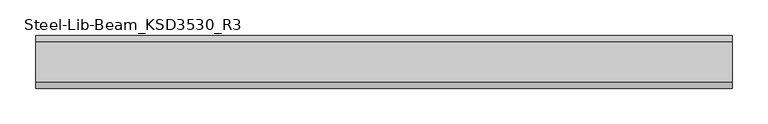
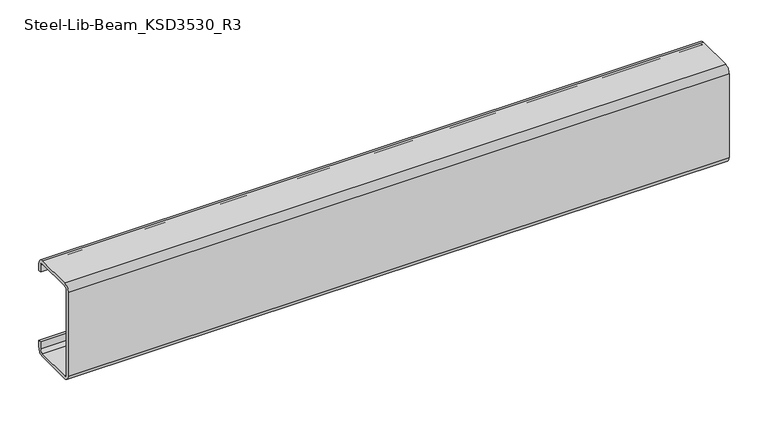
"""IFC4 building model written with IfcOpenShell, lengths in millimetres: beam geometry, Steel-Lib-Beam_KSD3530_R3 : BMS291_C-150×75x20x4.5."""

from ifc_helpers import new_model, si_unit, point, frame, frame_2d, origin, place, context, project, spatial, polyline, circle_curve, trimmed, segment, composite_curve, outline, extrude, source, transform, mapped, element, save


def steel_lib_beam_ksd3530_r3_6a3dd1c6(model_context):
    return source(origin(), model_context, "Body", "SweptSolid", [
        extrude(outline(composite_curve([segment(polyline([(50.0, 66.0), (50.0, 55.0), (45.5, 55.0), (45.5, 66.0)]), True, "CONTINUOUS"), segment(trimmed(circle_curve(frame_2d((41.0, 66.0)), 4.5), [point((45.5, 66.0))], [point((41.0, 70.5))], True, "CARTESIAN"), True, "CONTINUOUS"), segment(polyline([(41.0, 70.5), (-16.0, 70.5)]), True, "CONTINUOUS"), segment(trimmed(circle_curve(frame_2d((-16.0, 66.0)), 4.5), [point((-16.0, 70.5))], [point((-20.5, 66.0))], True, "CARTESIAN"), True, "CONTINUOUS"), segment(polyline([(-20.5, 66.0), (-20.5, -66.0)]), True, "CONTINUOUS"), segment(trimmed(circle_curve(frame_2d((-16.0, -66.0)), 4.5), [point((-20.5, -66.0))], [point((-16.0, -70.5))], True, "CARTESIAN"), True, "CONTINUOUS"), segment(polyline([(-16.0, -70.5), (41.0, -70.5)]), True, "CONTINUOUS"), segment(trimmed(circle_curve(frame_2d((41.0, -66.0)), 4.5), [point((41.0, -70.5))], [point((45.5, -66.0))], True, "CARTESIAN"), True, "CONTINUOUS"), segment(polyline([(45.5, -66.0), (45.5, -55.0), (50.0, -55.0), (50.0, -66.0)]), True, "CONTINUOUS"), segment(trimmed(circle_curve(frame_2d((41.0, -66.0)), 9.0), [point((50.0, -66.0))], [point((41.0, -75.0))], False, "CARTESIAN"), True, "CONTINUOUS"), segment(polyline([(41.0, -75.0), (-16.0, -75.0)]), True, "CONTINUOUS"), segment(trimmed(circle_curve(frame_2d((-16.0, -66.0)), 9.0), [point((-16.0, -75.0))], [point((-25.0, -66.0))], False, "CARTESIAN"), True, "CONTINUOUS"), segment(polyline([(-25.0, -66.0), (-25.0, 66.0)]), True, "CONTINUOUS"), segment(trimmed(circle_curve(frame_2d((-16.0, 66.0)), 9.0), [point((-25.0, 66.0))], [point((-16.0, 75.0))], False, "CARTESIAN"), True, "CONTINUOUS"), segment(polyline([(-16.0, 75.0), (41.0, 75.0)]), True, "CONTINUOUS"), segment(trimmed(circle_curve(frame_2d((41.0, 66.0)), 9.0), [point((41.0, 75.0))], [point((50.0, 66.0))], False, "CARTESIAN"), True, "CONTINUOUS")], self_intersect=False)), frame((-490.0, 0.0, 0.0), z_axis=(1.0, 0.0, 0.0), x_axis=(0.0, 1.0, 0.0)), (0.0, 0.0, 1.0), 980.0),
    ])


if __name__ == "__main__":
    model = new_model("IFC4")
    model_context = context("Model", 3, world=origin())
    ifc_project = project(units=[si_unit("LENGTHUNIT", "METRE", prefix="MILLI")], contexts=[model_context])
    site = spatial("IfcSite", under=ifc_project)
    building = spatial("IfcBuilding", under=site)
    placement = place(None, origin())
    steel_lib_beam_ksd3530_r3_shape = steel_lib_beam_ksd3530_r3_6a3dd1c6(model_context)
    element("IfcBeam", 1, ObjectType="Steel-Lib-Beam_KSD3530_R3 : BMS291_C-150×75x20x4.5", at=placement, inside=building, context=model_context, shape_type="MappedRepresentation", body=[
        mapped(steel_lib_beam_ksd3530_r3_shape, transform((0.0, 0.0, 0.0), x_axis=(1.0, 0.0, 0.0), y_axis=(0.0, 1.0, 0.0), z_axis=(0.0, 0.0, 1.0))),
    ])
    save(model, "model.ifc")

# Revit data of these elements
# Type "Steel-Lib-Beam_KSD3530_R3 : BMS291_C-150×75x20x4.5"
#   Keynote = "C-150×75x20x4.5"
#   SteelWeight = "Light"
#   x = 0.0250 m
#   t1 = 0.0090 m
#   t = 0.0045 m
#   Surface Area = 0.629834 m²/m
#   Section Area = 13.9688 cm²
#   Mass per Unit Length = 10.9655 kg/m
#   C = 0.0200 m
#   A = 0.0750 m
#   Length [instance default] = 1.5000 m
#   H = 0.1500 m
#   hec_material4 [instance default] = none
#   hec_material3 [instance default] = none
#   hec_material2 [instance default] = none
#   hec_material1 [instance default] = none
#   Structural Material [instance default] = Metal - Steel - Light Gauge
#   Assembly Code = ""
# Element 1 (IfcBeam, "Steel-Lib-Beam_KSD3530_R3 : BMS291_C-150×75x20x4.5")
#   Structural Material = none
# Materials
#   "Metal - Steel - Light Gauge": class "Metal", colour RGB 247 247 247, transparency 0
